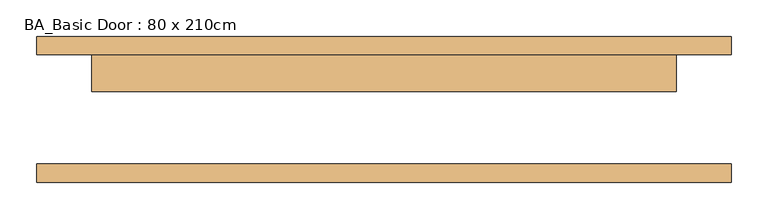
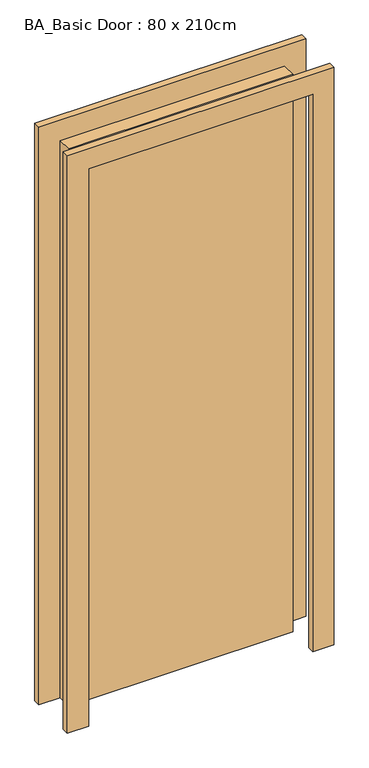
"""IFC4 building model written with IfcOpenShell, lengths in millimetres: door geometry, BA_Basic Door : 80 x 210cm."""

import ifcopenshell
import ifcopenshell.guid

model = None  # the IFC model being written
_history = None  # IfcOwnerHistory: only IFC2X3 demands one
_inside = {}  # id of a spatial element -> (the spatial element, [elements in it])
_under = {}  # id of a project, library or spatial element -> (it, [spatial elements below it])
_declared = {}  # id of a project -> (the project, [libraries it declares])
_typed = {}  # id of a type object -> (the type object, [elements of that type])
_made_of = {}  # id of a material, layer set ... -> (it, [elements and type objects made of it])


def new_model(schema):
    """Start an empty IFC model of exactly this schema.

    Asked for "IFC4X3", IfcOpenShell would pick the latest addendum, in which some entities
    have other attributes; the version numbers below select the first issue.
    IFC2X3 requires an IfcOwnerHistory on every rooted entity: one is made here for all.
    """
    global model, _history
    if schema == "IFC4X3":
        model = ifcopenshell.file(schema_version=(4, 3, 0, 0))
    else:
        model = ifcopenshell.file(schema=schema)
    _inside.clear()
    _under.clear()
    _declared.clear()
    _typed.clear()
    _made_of.clear()
    _history = None
    if model.schema == "IFC2X3":
        org = make("IfcOrganization", Name="unknown")
        user = make(
            "IfcPersonAndOrganization",
            ThePerson=make("IfcPerson", FamilyName="unknown"),
            TheOrganization=org,
        )
        app = make(
            "IfcApplication",
            ApplicationDeveloper=org,
            Version="unknown",
            ApplicationFullName="unknown",
            ApplicationIdentifier="unknown",
        )
        _history = make(
            "IfcOwnerHistory",
            OwningUser=user,
            OwningApplication=app,
            ChangeAction="ADDED",
            CreationDate=0,
        )
    return model


def make(cls, **values):
    """One entity of the class cls with the attributes given. An attribute that is None is left unset."""
    return model.create_entity(
        cls, **{name: value for name, value in values.items() if value is not None}
    )


def rooted(cls, **values):
    """An entity with a GlobalId (a new one), such as an element, a storey or a relation."""
    return make(cls, GlobalId=ifcopenshell.guid.new(), OwnerHistory=_history, **values)


def si_unit(unit_type, name, prefix=None):
    """IfcSIUnit, for example si_unit("LENGTHUNIT", "METRE", prefix="MILLI")."""
    return make("IfcSIUnit", UnitType=unit_type, Prefix=prefix, Name=name)


def assignment(units):
    """IfcUnitAssignment: the units of a project."""
    return None if units is None else make("IfcUnitAssignment", Units=units)


def point(xyz):
    """IfcCartesianPoint."""
    return None if xyz is None else make("IfcCartesianPoint", Coordinates=xyz)


def direction(xyz):
    """IfcDirection."""
    return None if xyz is None else make("IfcDirection", DirectionRatios=xyz)


def frame(location, z_axis=None, x_axis=None):
    """IfcAxis2Placement3D, a coordinate frame: its origin and axes. An axis left out is left unset."""
    return make(
        "IfcAxis2Placement3D",
        Location=point(location),
        Axis=direction(z_axis),
        RefDirection=direction(x_axis),
    )


def origin():
    """The frame at (0, 0, 0) with its axes left unset."""
    return frame((0.0, 0.0, 0.0))


def origin_with_axes():
    """The frame at (0, 0, 0) with the z axis (0, 0, 1) and the x axis (1, 0, 0) written out."""
    return frame((0.0, 0.0, 0.0), z_axis=(0.0, 0.0, 1.0), x_axis=(1.0, 0.0, 0.0))


def place(relative_to, where):
    """IfcLocalPlacement: puts the frame where relative to a parent placement (None: the world)."""
    return make(
        "IfcLocalPlacement", PlacementRelTo=relative_to, RelativePlacement=where
    )


def context(
    kind, dimensions, precision=None, world=None, true_north=None, identifier=None
):
    """IfcGeometricRepresentationContext, for example the 3D "Model" context."""
    return make(
        "IfcGeometricRepresentationContext",
        ContextIdentifier=identifier,
        ContextType=kind,
        CoordinateSpaceDimension=dimensions,
        Precision=precision,
        WorldCoordinateSystem=world,
        TrueNorth=true_north,
    )


def project(units=None, contexts=None):
    """IfcProject with its units and contexts."""
    return rooted(
        "IfcProject",
        Name="project",
        RepresentationContexts=contexts,
        UnitsInContext=assignment(units),
    )


def spatial(cls, under=None, at=None, **own):
    """A site, building, storey or space (cls), placed at a placement, below another one or the project."""
    s = rooted(cls, ObjectPlacement=at, **own)
    if under is not None:
        _under.setdefault(under.id(), (under, []))[1].append(s)
    return s


def polyline(points):
    """IfcPolyline through the points."""
    return make("IfcPolyline", Points=[point(p) for p in points])


def outline(outer, holes=None, kind="AREA"):
    """IfcArbitraryClosedProfileDef: a profile drawn as a closed curve; with holes, ...WithVoids."""
    if holes is None:
        return make("IfcArbitraryClosedProfileDef", ProfileType=kind, OuterCurve=outer)
    return make(
        "IfcArbitraryProfileDefWithVoids",
        ProfileType=kind,
        OuterCurve=outer,
        InnerCurves=holes,
    )


def extrude(swept, where, along, depth):
    """IfcExtrudedAreaSolid: the profile swept, set in the frame where, extruded along a direction by depth."""
    return make(
        "IfcExtrudedAreaSolid",
        SweptArea=swept,
        Position=where,
        ExtrudedDirection=direction(along),
        Depth=depth,
    )


def shape(context_of_items, identifier, shape_type, items):
    """IfcShapeRepresentation: the items that make up one representation, for example the "Body"."""
    return make(
        "IfcShapeRepresentation",
        ContextOfItems=context_of_items,
        RepresentationIdentifier=identifier,
        RepresentationType=shape_type,
        Items=items,
    )


def source(mapping_origin, context_of_items, identifier, shape_type, items):
    """IfcRepresentationMap: a shape defined once, which mapped items show again and again."""
    return make(
        "IfcRepresentationMap",
        MappingOrigin=mapping_origin,
        MappedRepresentation=shape(context_of_items, identifier, shape_type, items),
    )


def transform(
    local_origin,
    x_axis=None,
    y_axis=None,
    z_axis=None,
    scale=None,
    scale2=None,
    scale3=None,
    uniform=True,
):
    """IfcCartesianTransformationOperator3D, or its non-uniform kind. x_axis, y_axis, z_axis: its Axis1, 2, 3."""
    if uniform:
        return make(
            "IfcCartesianTransformationOperator3D",
            Axis1=direction(x_axis),
            Axis2=direction(y_axis),
            LocalOrigin=point(local_origin),
            Scale=scale,
            Axis3=direction(z_axis),
        )
    return make(
        "IfcCartesianTransformationOperator3DnonUniform",
        Axis1=direction(x_axis),
        Axis2=direction(y_axis),
        LocalOrigin=point(local_origin),
        Scale=scale,
        Axis3=direction(z_axis),
        Scale2=scale2,
        Scale3=scale3,
    )


def mapped(mapping_source, mapping_target):
    """IfcMappedItem: shows the shape of a source again, moved by a transform."""
    return make(
        "IfcMappedItem", MappingSource=mapping_source, MappingTarget=mapping_target
    )


def made_of(thing, what):
    """Note that an element or type object is made of a material, layer set ...; save() writes the relation."""
    if what is not None:
        _made_of.setdefault(what.id(), (what, []))[1].append(thing)
    return thing


def element(
    cls,
    number,
    at=None,
    inside=None,
    cuts=None,
    type_object=None,
    material=None,
    context=None,
    identifier="Body",
    shape_type=None,
    held_by="IfcProductDefinitionShape",
    body=None,
    shapes=None,
    **own,
):
    """One element of the class cls, such as IfcWall. Its Tag is "e" and its number.

    at: its placement. inside: the storey or other place that contains it. cuts: it is an
    opening in that element (IfcRelVoidsElement). A single representation is given by context,
    identifier, shape_type and body (its items); several are given by shapes. held_by: the class
    of the entity that holds the representations. save() writes the other relations.
    """
    e = rooted(cls, Tag="e%d" % number, ObjectPlacement=at, **own)
    if body is not None:
        shapes = [shape(context, identifier, shape_type, body)]
    if shapes is not None:
        e.Representation = make(held_by, Representations=shapes)
    if inside is not None:
        _inside.setdefault(inside.id(), (inside, []))[1].append(e)
    if cuts is not None:
        rooted(
            "IfcRelVoidsElement", RelatingBuildingElement=cuts, RelatedOpeningElement=e
        )
    if type_object is not None:
        _typed.setdefault(type_object.id(), (type_object, []))[1].append(e)
    return made_of(e, material)


def aggregate(whole, parts):
    """IfcRelAggregates: a whole, such as a stair, and the parts it consists of."""
    return rooted("IfcRelAggregates", RelatingObject=whole, RelatedObjects=parts)


def save(model, path):
    """Write the relations noted so far, then the file.

    IfcRelAggregates (storeys below a building ...), IfcRelContainedInSpatialStructure (elements
    in a storey), IfcRelDefinesByType, IfcRelAssociatesMaterial and IfcRelDeclares: one each for
    every whole, place, type object, material and project.
    """
    for whole, parts in _under.values():
        aggregate(whole, parts)
    for where, things in _inside.values():
        rooted(
            "IfcRelContainedInSpatialStructure",
            RelatedElements=things,
            RelatingStructure=where,
        )
    for kind, things in _typed.values():
        rooted("IfcRelDefinesByType", RelatedObjects=things, RelatingType=kind)
    for what, things in _made_of.values():
        rooted("IfcRelAssociatesMaterial", RelatedObjects=things, RelatingMaterial=what)
    for by, libraries in _declared.values():
        rooted("IfcRelDeclares", RelatingContext=by, RelatedDefinitions=libraries)
    model.write(path)


def ba_basic_door_80_x_210cm_4d281df6(model_context):
    return source(origin(), model_context, "Body", "SweptSolid", [
        extrude(outline(polyline([(400.0, 24.0), (-400.0, 24.0), (-400.0, 75.0), (400.0, 75.0), (400.0, 24.0)])), origin_with_axes(), (0.0, 0.0, 1.0), 2100.0),
        extrude(outline(polyline([(2176.0, -476.0), (0.0, -476.0), (0.0, -400.0), (2100.0, -400.0), (2100.0, 400.0), (0.0, 400.0), (0.0, 476.0), (2176.0, 476.0), (2176.0, -476.0)])), frame((0.0, 75.0, 0.0), z_axis=(0.0, 1.0, 0.0), x_axis=(0.0, 0.0, 1.0)), (0.0, 0.0, 1.0), 25.0),
        extrude(outline(polyline([(2176.0, 476.0), (2176.0, -476.0), (0.0, -476.0), (0.0, -400.0), (2100.0, -400.0), (2100.0, 400.0), (0.0, 400.0), (0.0, 476.0), (2176.0, 476.0)])), frame((0.0, -100.0, 0.0), z_axis=(0.0, 1.0, 0.0), x_axis=(0.0, 0.0, 1.0)), (0.0, 0.0, 1.0), 25.0),
    ])


if __name__ == "__main__":
    model = new_model("IFC4")
    model_context = context("Model", 3, world=origin())
    ifc_project = project(units=[si_unit("LENGTHUNIT", "METRE", prefix="MILLI")], contexts=[model_context])
    site = spatial("IfcSite", under=ifc_project)
    building = spatial("IfcBuilding", under=site)
    placement = place(None, origin())
    ba_basic_door_80_x_210cm_shape = ba_basic_door_80_x_210cm_4d281df6(model_context)
    element("IfcDoor", 1, ObjectType="BA_Basic Door : 80 x 210cm", at=placement, inside=building, context=model_context, shape_type="MappedRepresentation", body=[
        mapped(ba_basic_door_80_x_210cm_shape, transform((0.0, 0.0, 0.0), x_axis=(1.0, 0.0, 0.0), y_axis=(0.0, 1.0, 0.0), z_axis=(0.0, 0.0, 1.0))),
    ])
    save(model, "model.ifc")

# Revit data of these elements
# Type "BA_Basic Door : 80 x 210cm"
#   Type Mark = "41"
#   Construction Type Id = "MDOOR"
#   Analytic Construction = "Metal"
#   Window height [instance default] = 1000 mm
#   Thickness = 51 mm
#   Thermal Resistance (R) = 0.270117 (m²·K)/W
#   Cut [instance default] = -100 mm
#   Heat Transfer Coefficient (U) = 3.7021 W/(m²·K)
#   Height = 2100 mm
#   Trim Projection Ext = 25 mm
#   Trim Projection Int = 25 mm
#   Trim Width = 76 mm
#   Width = 800 mm
#   Door window [instance default] = no
#   Define Thermal Properties by = 1
#   Door Material = Default
#   Frame Material = Default
#   Visual Light Transmittance = 0
#   Solar Heat Gain Coefficient = 0
#   Function = (empty or 0)
#   Wall Closure = (empty or 0)
# Element 1 (IfcDoor, "BA_Basic Door : 80 x 210cm")
#   Materials on its faces: "Default"
# Materials
#   "Default": class "Generic", colour RGB 255 255 255, transparency 0, Cost = 0
